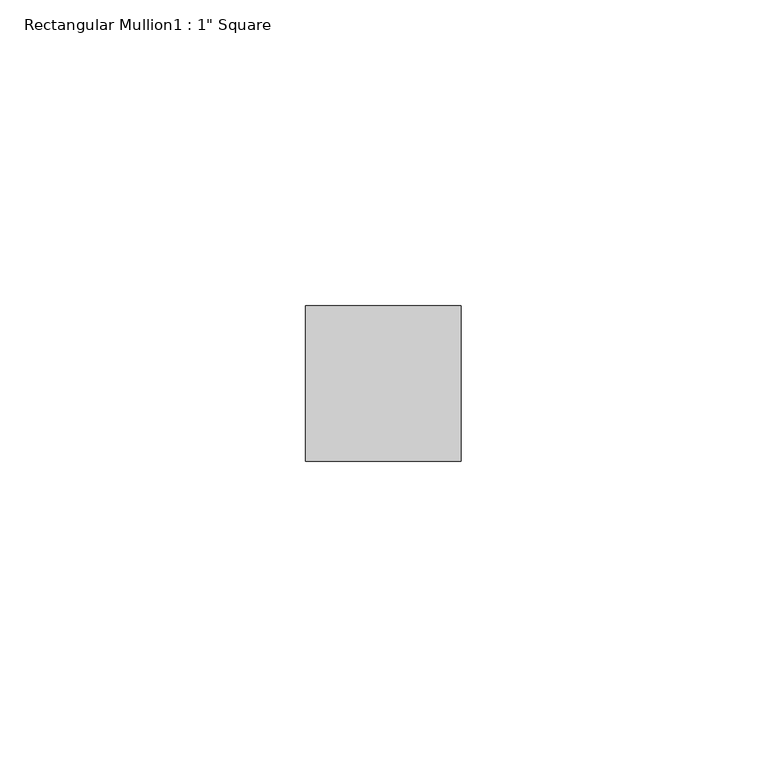
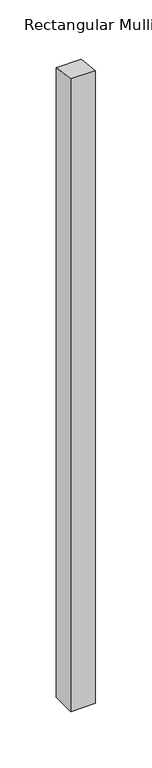
"""IFC4 building model written with IfcOpenShell, lengths in millimetres: member geometry."""

from ifc_helpers import new_model, si_unit, frame, origin, place, context, project, spatial, polyline, outline, extrude, source, transform, mapped, element, save


def member_e06bcec6(model_context):
    return source(origin(), model_context, "Body", "SweptSolid", [
        extrude(outline(polyline([(-44.45, 5.6588474), (-19.05, 2.4252203), (-19.05, -680.0402655), (-44.45, -680.0402655), (-44.45, 5.6588474)])), frame((-25.4, 0.0, 0.0), z_axis=(1.0, 0.0, 0.0), x_axis=(0.0, 1.0, 0.0)), (0.0, 0.0, 1.0), 25.4),
    ])


if __name__ == "__main__":
    model = new_model("IFC4")
    model_context = context("Model", 3, world=origin())
    ifc_project = project(units=[si_unit("LENGTHUNIT", "METRE", prefix="MILLI")], contexts=[model_context])
    site = spatial("IfcSite", under=ifc_project)
    building = spatial("IfcBuilding", under=site)
    placement = place(None, origin())
    member_shape = member_e06bcec6(model_context)
    element("IfcMember", 1, ObjectType="Rectangular Mullion1 : 1\" Square", at=placement, inside=building, context=model_context, shape_type="MappedRepresentation", body=[
        mapped(member_shape, transform((0.0, 0.0, 0.0), x_axis=(1.0, 0.0, 0.0), y_axis=(0.0, 1.0, 0.0), z_axis=(0.0, 0.0, 1.0))),
    ])
    save(model, "model.ifc")

# Revit data of these elements
# Type "Rectangular Mullion1 : 1\" Square"
#   built-in parameter 1007351 = 0.104167 (stored number, unit not read)
#   built-in parameter 1007304 = 0.0833333 (stored number, unit not read)
#   built-in parameter 1007301 = 0.0416667 (stored number, unit not read)
#   built-in parameter 1007300 = 0.0416667 (stored number, unit not read)
